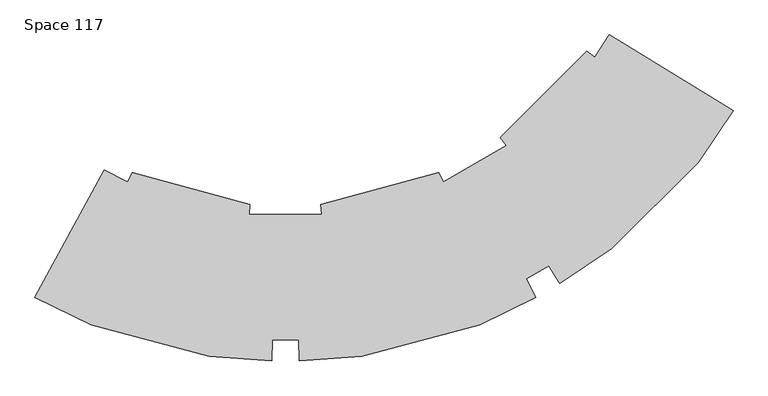
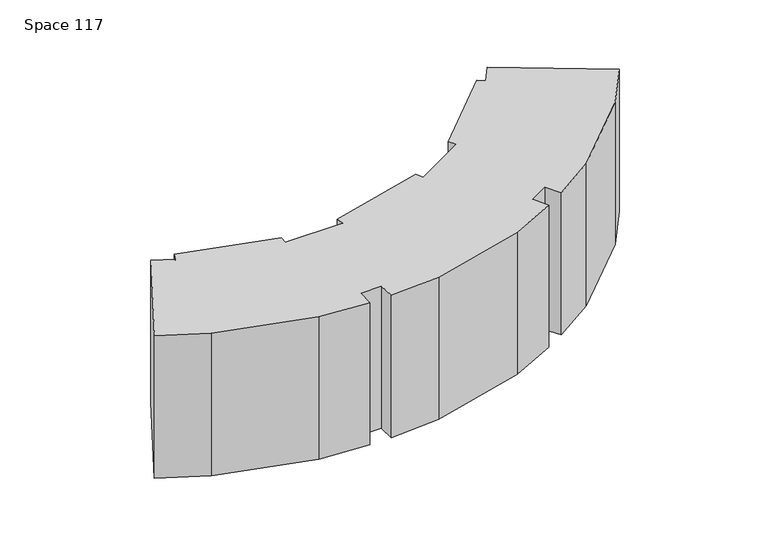
"""IFC4 building model written with IfcOpenShell, lengths in millimetres: proxy geometry, Space 117."""

from ifc_helpers import new_model, si_unit, point, frame_2d, origin, origin_with_axes, place, context, project, spatial, polyline, circle_curve, trimmed, segment, composite_curve, outline, extrude, source, transform, mapped, element, save


def space_117_2c79f81d(model_context):
    return source(origin(), model_context, "Body", "SweptSolid", [
        extrude(outline(composite_curve([segment(polyline([(-27087.4912586, -31539.0895707), (-25205.3245192, -32043.4146285), (-25220.7766392, -32203.891031)]), True, "CONTINUOUS"), segment(trimmed(circle_curve(frame_2d((-24639.5440345, -26167.559635)), 6064.25), [point((-25220.7766392, -32203.891031))], [point((-24058.3114298, -32203.891031))], True, "CARTESIAN"), True, "CONTINUOUS"), segment(polyline([(-24058.3114298, -32203.891031), (-24073.7635498, -32043.4146285), (-22191.5968104, -31539.0895707), (-22124.7405377, -31685.7922719)]), True, "CONTINUOUS"), segment(trimmed(circle_curve(frame_2d((-24639.5440345, -26167.559635)), 6064.25), [point((-22124.7405377, -31685.7922719))], [point((-21118.0161353, -31104.5596672))], True, "CARTESIAN"), True, "CONTINUOUS"), segment(polyline([(-21118.0161353, -31104.5596672), (-21211.6362651, -30973.309086), (-19833.7945835, -29595.4674045), (-19702.5440023, -29689.0875342)]), True, "CONTINUOUS"), segment(trimmed(circle_curve(frame_2d((-24639.5440345, -26167.559635)), 6064.25), [point((-19702.5440023, -29689.0875342))], [point((-19468.9209178, -29336.1215561))], True, "CARTESIAN"), True, "CONTINUOUS"), segment(polyline([(-19468.9209178, -29336.1215561), (-17496.6519385, -30544.7295411), (-18055.7038715, -31373.5581164), (-19433.5455531, -32751.399798), (-20262.3741285, -33310.4517311), (-20435.807957, -33027.4334453)]), True, "CONTINUOUS"), segment(trimmed(circle_curve(frame_2d((-24639.5440345, -26167.559635)), 8045.45), [point((-20435.807957, -33027.4334453))], [point((-20800.5870868, -33238.0387741))], False, "CARTESIAN"), True, "CONTINUOUS"), segment(polyline([(-20800.5870868, -33238.0387741), (-20642.2029759, -33529.7460184), (-21540.7704396, -33968.0066535), (-23422.937179, -34472.3317113), (-24420.2497472, -34542.0705997), (-24428.9387057, -34210.2526602)]), True, "CONTINUOUS"), segment(trimmed(circle_curve(frame_2d((-24639.5440345, -26167.559635)), 8045.45), [point((-24428.9387057, -34210.2526602))], [point((-24850.1493633, -34210.2526602))], False, "CARTESIAN"), True, "CONTINUOUS"), segment(polyline([(-24850.1493633, -34210.2526602), (-24858.8383218, -34542.0705997), (-25856.15089, -34472.3317113), (-27738.3176294, -33968.0066535), (-28636.8850931, -33529.7460184), (-27533.1540464, -31496.9263105)]), True, "CONTINUOUS"), segment(trimmed(circle_curve(frame_2d((-24639.5440345, -26167.559635)), 6064.25), [point((-27533.1540464, -31496.9263105))], [point((-27154.3475313, -31685.7922719))], True, "CARTESIAN"), True, "CONTINUOUS"), segment(polyline([(-27154.3475313, -31685.7922719), (-27087.4912586, -31539.0895707)]), True, "CONTINUOUS")], self_intersect=False)), origin_with_axes(), (0.0, 0.0, 1.0), 3048.0),
    ])


if __name__ == "__main__":
    model = new_model("IFC4")
    model_context = context("Model", 3, world=origin())
    ifc_project = project(units=[si_unit("LENGTHUNIT", "METRE", prefix="MILLI")], contexts=[model_context])
    site = spatial("IfcSite", under=ifc_project)
    building = spatial("IfcBuilding", under=site)
    placement = place(None, origin())
    space_117_shape = space_117_2c79f81d(model_context)
    element("IfcBuildingElementProxy", 1, Name="Space 117", ObjectType="Space 117", at=placement, inside=building, context=model_context, shape_type="MappedRepresentation", body=[
        mapped(space_117_shape, transform((0.0, 0.0, 0.0), x_axis=(1.0, 0.0, 0.0), y_axis=(0.0, 1.0, 0.0), z_axis=(0.0, 0.0, 1.0))),
    ])
    save(model, "model.ifc")

# Revit data of these elements
# Element 1 (IfcBuildingElementProxy, "Space 117")
#   Materials on its faces: "Render Material 255-255-255"
# Materials
#   "Render Material 255-255-255": class "Unassigned", colour RGB 255 255 255, transparency 0
